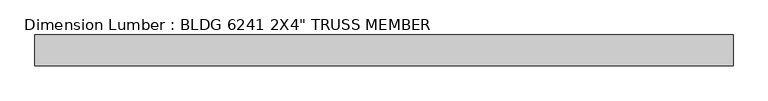
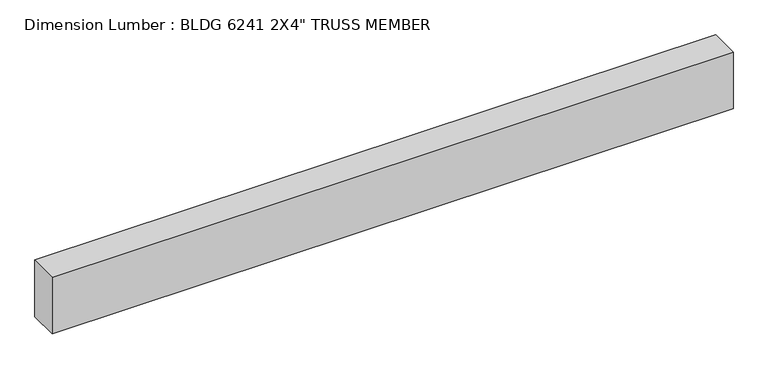
"""IFC4 building model written with IfcOpenShell, lengths in millimetres: beam geometry."""

from ifc_helpers import new_model, si_unit, frame, origin, place, context, project, spatial, polyline, outline, extrude, source, transform, mapped, element, save


def beam_5ac0b85f(model_context):
    return source(origin(), model_context, "Body", "SweptSolid", [
        extrude(outline(polyline([(571.5, -25.4), (-584.2, -25.4), (-584.2, 25.4), (571.5, 25.4), (571.5, -25.4)])), frame((0.0, 0.0, -50.8), z_axis=(0.0, 0.0, 1.0), x_axis=(1.0, 0.0, 0.0)), (0.0, 0.0, 1.0), 101.6),
    ])


if __name__ == "__main__":
    model = new_model("IFC4")
    model_context = context("Model", 3, world=origin())
    ifc_project = project(units=[si_unit("LENGTHUNIT", "METRE", prefix="MILLI")], contexts=[model_context])
    site = spatial("IfcSite", under=ifc_project)
    building = spatial("IfcBuilding", under=site)
    placement = place(None, origin())
    beam_shape = beam_5ac0b85f(model_context)
    element("IfcBeam", 1, ObjectType="Dimension Lumber : BLDG 6241 2X4\" TRUSS MEMBER", at=placement, inside=building, context=model_context, shape_type="MappedRepresentation", body=[
        mapped(beam_shape, transform((0.0, 0.0, 0.0), x_axis=(1.0, 0.0, 0.0), y_axis=(0.0, 1.0, 0.0), z_axis=(0.0, 0.0, 1.0))),
    ])
    save(model, "model.ifc")

# Revit data of these elements
# Type "Dimension Lumber : BLDG 6241 2X4\" TRUSS MEMBER"
#   Assembly Code = "B10"
#   A = 0.273472 SF
#   Length [instance default] = 5' - 0"
#   b = 0' - 2"
#   d = 0' - 4"
#   Structural Material [instance default] = Softwood, Lumber
# Element 1 (IfcBeam, "Dimension Lumber : BLDG 6241 2X4\" TRUSS MEMBER")
#   Materials on its faces: "Softwood, Lumber"
# Materials
#   "Softwood, Lumber": class "Wood", colour RGB 223 192 134, transparency 0, Description = "Pinus Echinata", Cost = 0
